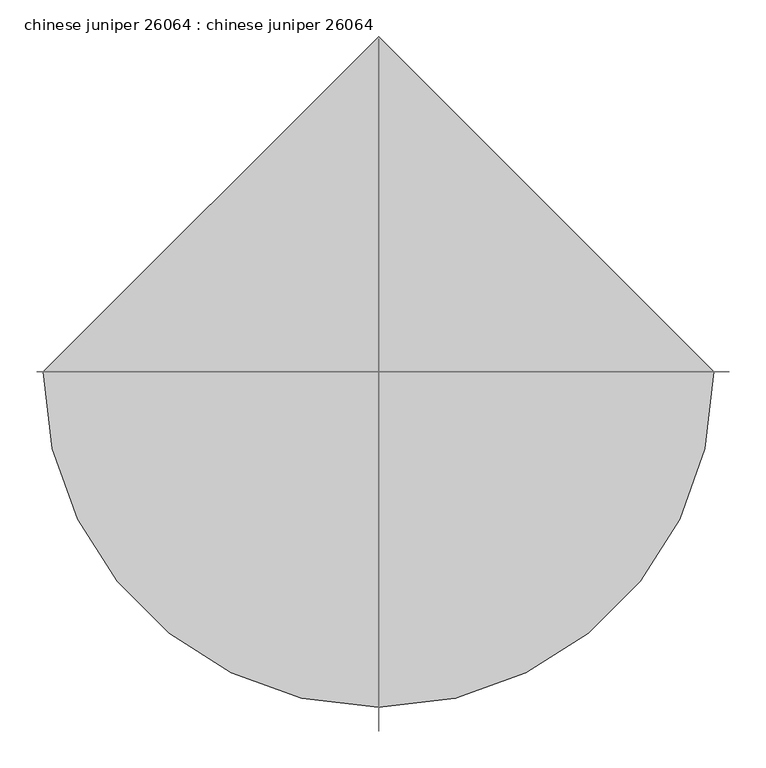
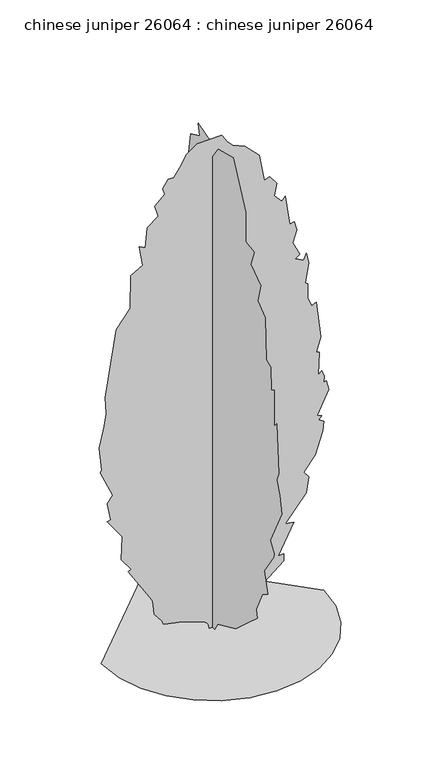
"""IFC4 building model written with IfcOpenShell, lengths in millimetres: proxy geometry, chinese juniper 26064 : chinese juniper 26064."""

from ifc_helpers import new_model, si_unit, origin, place, context, project, spatial, triangles, source, transform, mapped, element, save


def chinese_juniper_26064_chinese_juniper_26064_15d4aa58(model_context):
    return source(origin(), model_context, "Body", "Tessellation", [
        triangles([(-14.7143181, 6e-07, 1.3e-06), (-18.2037808, -3e-07, 17.9396969), (-27.6190332, -6e-07, 30.3914521), (-123.7652017, 1.5e-06, 65.7757953), (-201.8727252, 3.9e-06, 82.3498608), (-209.3591505, 3.1e-06, 101.0656516), (-239.5230251, 2.1e-06, 139.6788561), (-246.7912588, -1e-06, 198.3880905), (-258.0216416, -1.9e-06, 220.8470939), (-347.8566379, -6.4e-06, 363.0865585), (-336.2335828, -7.4e-06, 370.071561), (-375.982174, -8.9e-06, 425.7942498), (-371.9537135, -1.5e-05, 524.6285151), (-433.95022, -1.74e-05, 610.1379032), (-418.976897, -1.83e-05, 613.8793173), (-433.3685695, -2.22e-05, 689.5207758), (-411.4889457, -2.49e-05, 718.6876728), (-463.8943952, -2.95e-05, 834.7279736), (-456.4089872, -3.02e-05, 842.2133451), (-467.6383527, -3.58e-05, 943.2777431), (-447.3233863, -4.19e-05, 1031.4541197), (-437.6916704, -4.53e-05, 1081.7767748), (-441.4356279, -4.94e-05, 1152.8969976), (-396.5181298, -6.81e-05, 1433.6338589), (-340.3712663, -7.5e-05, 1508.4981846), (-337.3359501, -8.35e-05, 1648.2265743), (-287.9657986, -8.74e-05, 1676.941246), (-302.9391579, -9.18e-05, 1763.0323574), (-277.3841226, -9.21e-05, 1748.371479), (-269.2510252, -9.76e-05, 1834.1525803), (-224.3317467, -0.0001015, 1867.8406403), (-239.3045792, -0.0001038, 1916.5022049), (-198.1295307, -0.0001078, 1953.9342224), (-205.6159378, -0.000109, 1980.1369835), (-183.1569344, -0.000112, 2013.8251888), (-160.697931, -0.000113, 2013.8251888), (-134.9295457, -0.0001161, 2047.2821583), (-109.0956393, -0.0001202, 2095.8470718), (-62.7453116, -0.0001241, 2127.2339642), (36.9177479, -0.0001285, 2128.801165), (60.1491719, -0.0001273, 2092.4307106), (82.6081753, -0.000127, 2069.9720524), (132.5409287, -0.0001279, 2048.8239246), (191.1599888, -0.0001268, 1987.6224277), (213.6190104, -0.0001209, 1871.5845978), (236.0780138, -0.0001223, 1879.070042), (263.4699646, -0.0001212, 1839.8828991), (254.7932958, -0.0001178, 1789.2351185), (284.7399962, -0.0001171, 1755.5469131), (299.7107939, -0.0001186, 1770.5202724), (318.4281289, -0.0001119, 1643.2505699), (337.1429023, -0.0001129, 1646.9946728), (347.3206967, -0.0001111, 1609.9130699), (330.592212, -0.0001074, 1559.0291119), (359.6016332, -0.000105, 1497.2687828), (339.9877141, -0.0001034, 1485.5084541), (374.5749925, -0.0001038, 1467.3220642), (385.8043579, -0.0001059, 1493.5248253), (397.0337597, -0.0001037, 1448.6072182), (382.0629438, -9.81e-05, 1366.2577389), (392.870678, -9.81e-05, 1357.3651131), (391.3695342, -9.44e-05, 1296.562429), (408.2631251, -9.28e-05, 1257.7053532), (426.980442, -9.41e-05, 1265.1907974), (445.6952153, -8.55e-05, 1107.9794632), (426.980442, -8.11e-05, 1048.0886421), (438.6365255, -8.14e-05, 1044.1287821), (434.4658499, -7.54e-05, 947.0217007), (449.4392092, -7.68e-05, 958.2511024), (460.6685746, -7.57e-05, 932.0483414), (456.9246171, -7.4e-05, 905.8481964), (468.1539825, -7.47e-05, 909.5896105), (479.383348, -7.27e-05, 868.4161062), (430.7218924, -6.48e-05, 771.0931223), (449.4392092, -6.52e-05, 763.6077507), (438.2098074, -6.38e-05, 748.6343914), (456.9246171, -6.39e-05, 737.4049896), (452.9875754, -6.13e-05, 697.0620306), (423.2364844, -5.44e-05, 602.6499518), (374.5749925, -4.87e-05, 542.7590944), (397.0337597, -4.81e-05, 516.5563697), (384.7578738, -4.37e-05, 451.166393), (299.7107939, -3.36e-05, 344.3717488), (333.4014519, -3.49e-05, 340.6277913), (269.7666369, -2.47e-05, 217.1038994), (292.2254042, -2.57e-05, 217.1038994), (292.2254042, -2.39e-05, 187.1584707), (127.5256825, -8.7e-06, 52.4044321), (127.5256825, -9.8e-06, 71.1202274), (15.2310573, -7e-07, 0.0), (1.1e-06, 13.7891713, 0.00013), (2.6e-06, 34.4811189, 14.2963339), (5.1e-06, 77.4229995, 29.9456808), (7.2e-06, 178.488651, 67.3772736), (1.16e-05, 230.8930831, 116.0384931), (1.08e-05, 208.4340797, 119.7817057), (1.93e-05, 288.5449239, 235.2565704), (2.08e-05, 264.5824875, 291.9663175), (2.39e-05, 331.9587347, 389.2892833), (2.56e-05, 324.4733268, 434.2067814), (3.03e-05, 373.1322753, 494.0976388), (3.42e-05, 389.4924685, 565.7309481), (3.3e-05, 380.6202267, 640.0820784), (3.96e-05, 440.5110841, 729.9170746), (4.37e-05, 444.2524981, 819.7546143), (4.59e-05, 422.6319428, 893.2725832), (4.85e-05, 455.4818636, 1010.6565519), (4.9e-05, 425.5377248, 1051.8300562), (5.26e-05, 388.1056346, 1171.611771), (5.33e-05, 414.3083593, 1253.9613956), (5.72e-05, 384.3616407, 1373.7430378), (5.87e-05, 346.932094, 1444.8632607), (6.04e-05, 328.2147772, 1594.5917667), (5.89e-05, 305.75601, 1583.362365), (6.48e-05, 305.75601, 1718.1148956), (6.33e-05, 260.8385118, 1729.3441521), (6.18e-05, 237.0752094, 1809.303661), (6.41e-05, 223.406676, 1875.3287006), (6.41e-05, 178.488651, 1920.2461624), (6.9e-05, 156.0296476, 2055.0011639), (6.35e-05, 92.3955867, 2084.9454117), (6.6e-05, 102.0598133, 2133.1292439), (6.08e-05, 11.3487565, 2104.2112415), (6.18e-05, 6.3027505, 2040.0278046), (5.86e-05, -38.6152347, 2103.6627285), (5.52e-05, -147.1670527, 2133.606831), (4.72e-05, -237.0033388, 1950.1902649), (4.17e-05, -237.0033388, 1822.9231785), (3.86e-05, -296.2055936, 1812.3847229), (3.68e-05, -270.691199, 1744.3175114), (3.55e-05, -342.8426634, 1695.0642677), (3.29e-05, -323.0966666, 1617.050425), (2.88e-05, -375.4995727, 1575.8744499), (2.47e-05, -382.9874877, 1396.2018414), (2.28e-05, -413.5488853, 1383.1639744), (1.83e-05, -416.6756204, 1283.9081142), (1.8e-05, -439.1343876, 1298.8788574), (1.51e-05, -439.1343876, 1141.6675959), (1.12e-05, -457.849161, 1164.1263994), (5.4e-06, -472.8225203, 954.5096884), (4.6e-06, -456.5690065, 918.855542), (1.2e-06, -480.3104716, 864.672076), (1.4e-06, -491.5398371, 789.8078957), (-2.2e-06, -412.9316628, 628.8526766), (-5.3e-06, -439.1343876, 583.9351785), (-1.8e-06, -436.9195155, 568.0778978), (-3.2e-06, -368.0141647, 467.8974212), (-8.1e-06, -394.2168895, 381.8038754), (-7.5e-06, -353.0408054, 355.6011506), (-5.6e-06, -311.8672648, 265.7661362), (-7.4e-06, -319.3526728, 232.0767318), (-7.1e-06, -244.4894916, 164.6997216), (-6.7e-06, -165.8828434, 93.5794897), (-3.6e-06, -34.8715179, 33.6886368), (-3e-07, -16.1562041, 0.0001282), (-458.1641127, 0.0, 0.0001492), (-446.0508259, -104.9808196, 0.0001424), (-411.5549664, -201.3891246, 0.0001352), (-357.4375574, -286.4621113, 0.0001277), (-286.4621113, -357.4375574, 0.0001204), (-201.3891246, -411.5549664, 0.0001134), (-104.9808196, -446.0508259, 0.0001072), (2.06e-05, -458.1641127, 0.0001019), (104.9808196, -446.0508259, 9.8e-05), (201.3891246, -411.5549664, 9.58e-05), (286.4621113, -357.4375574, 9.54e-05), (357.4375574, -286.4621113, 9.65e-05), (411.5549664, -201.3888702, 9.92e-05), (446.0508259, -104.9808196, 0.0001034), (458.1641127, 4.01e-05, 0.0001092), (-5.98e-05, 458.1641127, 0.0001565)], [[57, 58, 59], [27, 28, 29], [87, 88, 89], [49, 50, 51], [13, 14, 15], [83, 84, 85], [74, 75, 76], [63, 64, 65], [68, 69, 70], [71, 72, 73], [9, 10, 11], [85, 86, 87], [85, 87, 89], [51, 52, 53], [54, 55, 56], [90, 1, 2], [66, 67, 68], [45, 46, 47], [17, 18, 19], [68, 70, 71], [45, 47, 48], [31, 32, 33], [76, 77, 78], [89, 90, 2], [89, 2, 3], [57, 59, 60], [51, 53, 54], [25, 26, 27], [39, 40, 41], [56, 57, 60], [71, 73, 74], [34, 35, 36], [33, 34, 36], [4, 5, 6], [60, 61, 62], [80, 81, 82], [38, 39, 41], [37, 38, 41], [37, 41, 42], [29, 30, 31], [15, 16, 17], [36, 37, 42], [33, 36, 42], [31, 33, 42], [31, 42, 43], [31, 43, 44], [31, 44, 45], [29, 31, 45], [29, 45, 48], [27, 29, 48], [25, 27, 48], [25, 48, 49], [25, 49, 51], [25, 51, 54], [25, 54, 56], [25, 56, 60], [25, 60, 62], [24, 25, 62], [23, 24, 62], [22, 23, 62], [22, 62, 63], [22, 63, 65], [22, 65, 66], [22, 66, 68], [21, 22, 68], [20, 21, 68], [19, 20, 68], [17, 19, 68], [17, 68, 71], [17, 71, 74], [15, 17, 74], [13, 15, 74], [13, 74, 76], [13, 76, 78], [13, 78, 79], [13, 79, 80], [12, 13, 80], [11, 12, 80], [9, 11, 80], [9, 80, 82], [9, 82, 83], [9, 83, 85], [9, 85, 89], [9, 89, 3], [9, 3, 4], [8, 9, 4], [8, 4, 6], [7, 8, 6], [138, 139, 140], [94, 95, 96], [136, 137, 138], [121, 122, 123], [112, 113, 114], [128, 129, 130], [121, 123, 124], [125, 126, 127], [124, 125, 127], [114, 115, 116], [147, 148, 149], [130, 131, 132], [124, 127, 128], [134, 135, 136], [154, 155, 91], [154, 91, 92], [150, 151, 152], [96, 97, 98], [119, 120, 121], [119, 121, 124], [119, 124, 128], [118, 119, 128], [117, 118, 128], [116, 117, 128], [116, 128, 130], [114, 116, 130], [114, 130, 132], [112, 114, 132], [112, 132, 133], [112, 133, 134], [112, 134, 136], [111, 112, 136], [110, 111, 136], [109, 110, 136], [109, 136, 138], [109, 138, 140], [109, 140, 141], [108, 109, 141], [107, 108, 141], [106, 107, 141], [105, 106, 141], [104, 105, 141], [103, 104, 141], [103, 141, 142], [103, 142, 143], [103, 143, 144], [102, 103, 144], [101, 102, 144], [100, 101, 144], [100, 144, 145], [100, 145, 146], [100, 146, 147], [100, 147, 149], [100, 149, 150], [100, 150, 152], [100, 152, 153], [100, 153, 154], [99, 100, 154], [98, 99, 154], [96, 98, 154], [96, 154, 92], [96, 92, 93], [96, 93, 94], [170, 171, 156], [169, 170, 156], [169, 156, 157], [168, 169, 157], [168, 157, 158], [168, 158, 159], [167, 168, 159], [166, 167, 159], [166, 159, 160], [166, 160, 161], [166, 161, 162], [166, 162, 163], [166, 163, 164], [166, 164, 165]], closed=False),
    ])


if __name__ == "__main__":
    model = new_model("IFC4")
    model_context = context("Model", 3, world=origin())
    ifc_project = project(units=[si_unit("LENGTHUNIT", "METRE", prefix="MILLI")], contexts=[model_context])
    site = spatial("IfcSite", under=ifc_project)
    building = spatial("IfcBuilding", under=site)
    placement = place(None, origin())
    chinese_juniper_26064_chinese_juniper_26064_shape = chinese_juniper_26064_chinese_juniper_26064_15d4aa58(model_context)
    element("IfcBuildingElementProxy", 1, Name="chinese juniper 26064 : chinese juniper 26064", ObjectType="chinese juniper 26064 : chinese juniper 26064", at=placement, inside=building, context=model_context, shape_type="MappedRepresentation", body=[
        mapped(chinese_juniper_26064_chinese_juniper_26064_shape, transform((0.0, 0.0, 0.0), x_axis=(1.0, 0.0, 0.0), y_axis=(0.0, 1.0, 0.0), z_axis=(0.0, 0.0, 1.0))),
    ])
    save(model, "model.ifc")

# Revit data of these elements
# Type "chinese juniper 26064 : chinese juniper 26064"
#   built-in parameter 1005195 = "RPC-16-FUM3-UUQ0-UBF0-N000-ST1L-LVER-AU"
#   Height = 0
